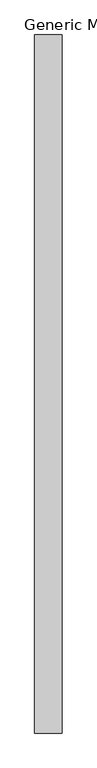
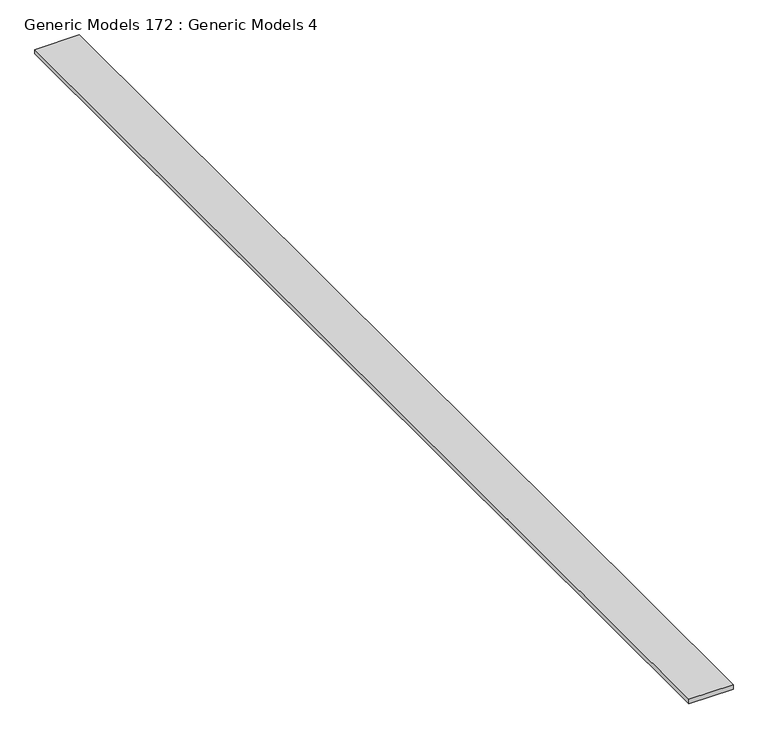
"""IFC4 building model written with IfcOpenShell, lengths in millimetres: proxy geometry, Generic Models 172 : Generic Models 4."""

from ifc_helpers import new_model, si_unit, frame, origin, place, context, project, spatial, polyline, outline, extrude, source, transform, mapped, element, save


def generic_models_172_generic_models_4_6759e7a3(model_context):
    return source(origin(), model_context, "Body", "SweptSolid", [
        extrude(outline(polyline([(-5937.4236296, -5493.3230338), (-6426.3736296, -5493.3230338), (-6426.3736296, 7054.2769662), (-5937.4236296, 7054.2769662), (-5937.4236296, -5493.3230338)])), frame((0.0, 0.0, 123005.596), z_axis=(0.0, 0.0, 1.0), x_axis=(1.0, 0.0, 0.0)), (0.0, 0.0, 1.0), 50.8),
    ])


if __name__ == "__main__":
    model = new_model("IFC4")
    model_context = context("Model", 3, world=origin())
    ifc_project = project(units=[si_unit("LENGTHUNIT", "METRE", prefix="MILLI")], contexts=[model_context])
    site = spatial("IfcSite", under=ifc_project)
    building = spatial("IfcBuilding", under=site)
    placement = place(None, origin())
    generic_models_172_generic_models_4_shape = generic_models_172_generic_models_4_6759e7a3(model_context)
    element("IfcBuildingElementProxy", 1, Name="Generic Models 172 : Generic Models 4", ObjectType="Generic Models 172 : Generic Models 4", at=placement, inside=building, context=model_context, shape_type="MappedRepresentation", body=[
        mapped(generic_models_172_generic_models_4_shape, transform((0.0, 0.0, 0.0), x_axis=(1.0, 0.0, 0.0), y_axis=(0.0, 1.0, 0.0), z_axis=(0.0, 0.0, 1.0))),
    ])
    save(model, "model.ifc")

# Revit data of these elements
# Element 1 (IfcBuildingElementProxy, "Generic Models 172 : Generic Models 4")
#   Materials on its faces: "_2\" SAND"
# Materials
#   "_2\" SAND": class "Generic", colour RGB 245 226 173, transparency 0, Cost = 0
